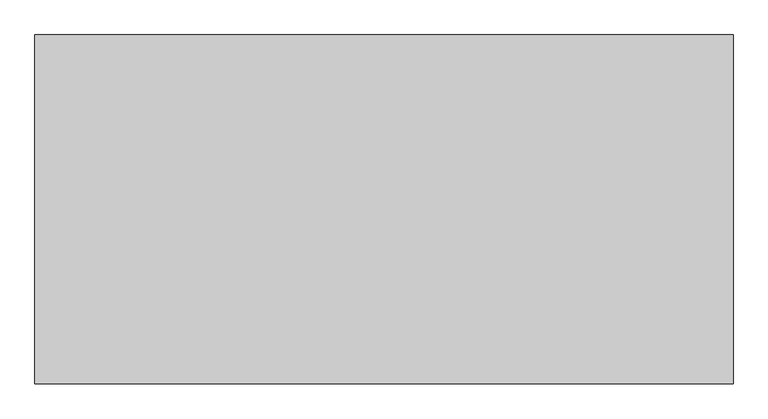
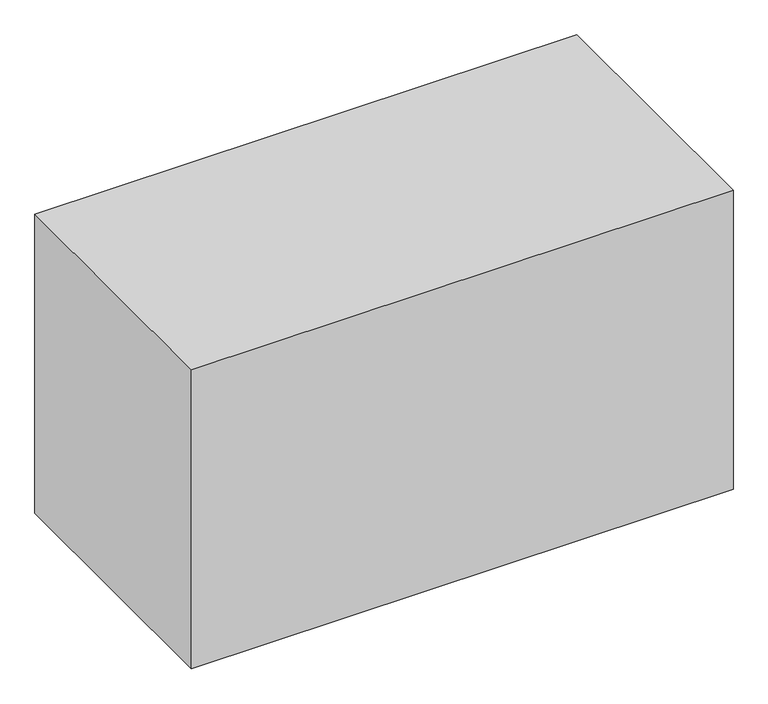
"""IFC4 building model written with IfcOpenShell, lengths in millimetres: proxy geometry, Space Planning Box_hec : Space Planning Box_hec."""

import ifcopenshell
import ifcopenshell.guid

model = None  # the IFC model being written
_history = None  # IfcOwnerHistory: only IFC2X3 demands one
_inside = {}  # id of a spatial element -> (the spatial element, [elements in it])
_under = {}  # id of a project, library or spatial element -> (it, [spatial elements below it])
_declared = {}  # id of a project -> (the project, [libraries it declares])
_typed = {}  # id of a type object -> (the type object, [elements of that type])
_made_of = {}  # id of a material, layer set ... -> (it, [elements and type objects made of it])


def new_model(schema):
    """Start an empty IFC model of exactly this schema.

    Asked for "IFC4X3", IfcOpenShell would pick the latest addendum, in which some entities
    have other attributes; the version numbers below select the first issue.
    IFC2X3 requires an IfcOwnerHistory on every rooted entity: one is made here for all.
    """
    global model, _history
    if schema == "IFC4X3":
        model = ifcopenshell.file(schema_version=(4, 3, 0, 0))
    else:
        model = ifcopenshell.file(schema=schema)
    _inside.clear()
    _under.clear()
    _declared.clear()
    _typed.clear()
    _made_of.clear()
    _history = None
    if model.schema == "IFC2X3":
        org = make("IfcOrganization", Name="unknown")
        user = make(
            "IfcPersonAndOrganization",
            ThePerson=make("IfcPerson", FamilyName="unknown"),
            TheOrganization=org,
        )
        app = make(
            "IfcApplication",
            ApplicationDeveloper=org,
            Version="unknown",
            ApplicationFullName="unknown",
            ApplicationIdentifier="unknown",
        )
        _history = make(
            "IfcOwnerHistory",
            OwningUser=user,
            OwningApplication=app,
            ChangeAction="ADDED",
            CreationDate=0,
        )
    return model


def make(cls, **values):
    """One entity of the class cls with the attributes given. An attribute that is None is left unset."""
    return model.create_entity(
        cls, **{name: value for name, value in values.items() if value is not None}
    )


def rooted(cls, **values):
    """An entity with a GlobalId (a new one), such as an element, a storey or a relation."""
    return make(cls, GlobalId=ifcopenshell.guid.new(), OwnerHistory=_history, **values)


def si_unit(unit_type, name, prefix=None):
    """IfcSIUnit, for example si_unit("LENGTHUNIT", "METRE", prefix="MILLI")."""
    return make("IfcSIUnit", UnitType=unit_type, Prefix=prefix, Name=name)


def assignment(units):
    """IfcUnitAssignment: the units of a project."""
    return None if units is None else make("IfcUnitAssignment", Units=units)


def point(xyz):
    """IfcCartesianPoint."""
    return None if xyz is None else make("IfcCartesianPoint", Coordinates=xyz)


def direction(xyz):
    """IfcDirection."""
    return None if xyz is None else make("IfcDirection", DirectionRatios=xyz)


def frame(location, z_axis=None, x_axis=None):
    """IfcAxis2Placement3D, a coordinate frame: its origin and axes. An axis left out is left unset."""
    return make(
        "IfcAxis2Placement3D",
        Location=point(location),
        Axis=direction(z_axis),
        RefDirection=direction(x_axis),
    )


def origin():
    """The frame at (0, 0, 0) with its axes left unset."""
    return frame((0.0, 0.0, 0.0))


def origin_with_axes():
    """The frame at (0, 0, 0) with the z axis (0, 0, 1) and the x axis (1, 0, 0) written out."""
    return frame((0.0, 0.0, 0.0), z_axis=(0.0, 0.0, 1.0), x_axis=(1.0, 0.0, 0.0))


def place(relative_to, where):
    """IfcLocalPlacement: puts the frame where relative to a parent placement (None: the world)."""
    return make(
        "IfcLocalPlacement", PlacementRelTo=relative_to, RelativePlacement=where
    )


def context(
    kind, dimensions, precision=None, world=None, true_north=None, identifier=None
):
    """IfcGeometricRepresentationContext, for example the 3D "Model" context."""
    return make(
        "IfcGeometricRepresentationContext",
        ContextIdentifier=identifier,
        ContextType=kind,
        CoordinateSpaceDimension=dimensions,
        Precision=precision,
        WorldCoordinateSystem=world,
        TrueNorth=true_north,
    )


def project(units=None, contexts=None):
    """IfcProject with its units and contexts."""
    return rooted(
        "IfcProject",
        Name="project",
        RepresentationContexts=contexts,
        UnitsInContext=assignment(units),
    )


def spatial(cls, under=None, at=None, **own):
    """A site, building, storey or space (cls), placed at a placement, below another one or the project."""
    s = rooted(cls, ObjectPlacement=at, **own)
    if under is not None:
        _under.setdefault(under.id(), (under, []))[1].append(s)
    return s


def polyline(points):
    """IfcPolyline through the points."""
    return make("IfcPolyline", Points=[point(p) for p in points])


def outline(outer, holes=None, kind="AREA"):
    """IfcArbitraryClosedProfileDef: a profile drawn as a closed curve; with holes, ...WithVoids."""
    if holes is None:
        return make("IfcArbitraryClosedProfileDef", ProfileType=kind, OuterCurve=outer)
    return make(
        "IfcArbitraryProfileDefWithVoids",
        ProfileType=kind,
        OuterCurve=outer,
        InnerCurves=holes,
    )


def extrude(swept, where, along, depth):
    """IfcExtrudedAreaSolid: the profile swept, set in the frame where, extruded along a direction by depth."""
    return make(
        "IfcExtrudedAreaSolid",
        SweptArea=swept,
        Position=where,
        ExtrudedDirection=direction(along),
        Depth=depth,
    )


def shape(context_of_items, identifier, shape_type, items):
    """IfcShapeRepresentation: the items that make up one representation, for example the "Body"."""
    return make(
        "IfcShapeRepresentation",
        ContextOfItems=context_of_items,
        RepresentationIdentifier=identifier,
        RepresentationType=shape_type,
        Items=items,
    )


def source(mapping_origin, context_of_items, identifier, shape_type, items):
    """IfcRepresentationMap: a shape defined once, which mapped items show again and again."""
    return make(
        "IfcRepresentationMap",
        MappingOrigin=mapping_origin,
        MappedRepresentation=shape(context_of_items, identifier, shape_type, items),
    )


def transform(
    local_origin,
    x_axis=None,
    y_axis=None,
    z_axis=None,
    scale=None,
    scale2=None,
    scale3=None,
    uniform=True,
):
    """IfcCartesianTransformationOperator3D, or its non-uniform kind. x_axis, y_axis, z_axis: its Axis1, 2, 3."""
    if uniform:
        return make(
            "IfcCartesianTransformationOperator3D",
            Axis1=direction(x_axis),
            Axis2=direction(y_axis),
            LocalOrigin=point(local_origin),
            Scale=scale,
            Axis3=direction(z_axis),
        )
    return make(
        "IfcCartesianTransformationOperator3DnonUniform",
        Axis1=direction(x_axis),
        Axis2=direction(y_axis),
        LocalOrigin=point(local_origin),
        Scale=scale,
        Axis3=direction(z_axis),
        Scale2=scale2,
        Scale3=scale3,
    )


def mapped(mapping_source, mapping_target):
    """IfcMappedItem: shows the shape of a source again, moved by a transform."""
    return make(
        "IfcMappedItem", MappingSource=mapping_source, MappingTarget=mapping_target
    )


def made_of(thing, what):
    """Note that an element or type object is made of a material, layer set ...; save() writes the relation."""
    if what is not None:
        _made_of.setdefault(what.id(), (what, []))[1].append(thing)
    return thing


def element(
    cls,
    number,
    at=None,
    inside=None,
    cuts=None,
    type_object=None,
    material=None,
    context=None,
    identifier="Body",
    shape_type=None,
    held_by="IfcProductDefinitionShape",
    body=None,
    shapes=None,
    **own,
):
    """One element of the class cls, such as IfcWall. Its Tag is "e" and its number.

    at: its placement. inside: the storey or other place that contains it. cuts: it is an
    opening in that element (IfcRelVoidsElement). A single representation is given by context,
    identifier, shape_type and body (its items); several are given by shapes. held_by: the class
    of the entity that holds the representations. save() writes the other relations.
    """
    e = rooted(cls, Tag="e%d" % number, ObjectPlacement=at, **own)
    if body is not None:
        shapes = [shape(context, identifier, shape_type, body)]
    if shapes is not None:
        e.Representation = make(held_by, Representations=shapes)
    if inside is not None:
        _inside.setdefault(inside.id(), (inside, []))[1].append(e)
    if cuts is not None:
        rooted(
            "IfcRelVoidsElement", RelatingBuildingElement=cuts, RelatedOpeningElement=e
        )
    if type_object is not None:
        _typed.setdefault(type_object.id(), (type_object, []))[1].append(e)
    return made_of(e, material)


def aggregate(whole, parts):
    """IfcRelAggregates: a whole, such as a stair, and the parts it consists of."""
    return rooted("IfcRelAggregates", RelatingObject=whole, RelatedObjects=parts)


def save(model, path):
    """Write the relations noted so far, then the file.

    IfcRelAggregates (storeys below a building ...), IfcRelContainedInSpatialStructure (elements
    in a storey), IfcRelDefinesByType, IfcRelAssociatesMaterial and IfcRelDeclares: one each for
    every whole, place, type object, material and project.
    """
    for whole, parts in _under.values():
        aggregate(whole, parts)
    for where, things in _inside.values():
        rooted(
            "IfcRelContainedInSpatialStructure",
            RelatedElements=things,
            RelatingStructure=where,
        )
    for kind, things in _typed.values():
        rooted("IfcRelDefinesByType", RelatedObjects=things, RelatingType=kind)
    for what, things in _made_of.values():
        rooted("IfcRelAssociatesMaterial", RelatedObjects=things, RelatingMaterial=what)
    for by, libraries in _declared.values():
        rooted("IfcRelDeclares", RelatingContext=by, RelatedDefinitions=libraries)
    model.write(path)


def generic_models_a5818909(model_context):
    return source(origin(), model_context, "Body", "SweptSolid", [
        extrude(outline(polyline([(3000.0, 1500.0), (3000.0, -1500.0), (-3000.0, -1500.0), (-3000.0, 1500.0), (3000.0, 1500.0)])), origin_with_axes(), (0.0, 0.0, 1.0), 3500.0),
    ])


if __name__ == "__main__":
    model = new_model("IFC4")
    model_context = context("Model", 3, world=origin())
    ifc_project = project(units=[si_unit("LENGTHUNIT", "METRE", prefix="MILLI")], contexts=[model_context])
    site = spatial("IfcSite", under=ifc_project)
    building = spatial("IfcBuilding", under=site)
    placement = place(None, origin())
    generic_models_shape = generic_models_a5818909(model_context)
    element("IfcBuildingElementProxy", 1, Name="Space Planning Box_hec : Space Planning Box_hec", ObjectType="Space Planning Box_hec : Space Planning Box_hec", at=placement, inside=building, context=model_context, shape_type="MappedRepresentation", body=[
        mapped(generic_models_shape, transform((0.0, 0.0, 0.0), x_axis=(1.0, 0.0, 0.0), y_axis=(0.0, 1.0, 0.0), z_axis=(0.0, 0.0, 1.0))),
    ])
    save(model, "model.ifc")

# Revit data of these elements
# Type "Space Planning Box_hec : Space Planning Box_hec"
#   Type Comments = "..."
#   Room Name [instance default] = "?"
#   Interior Finish [instance default] = ""
#   Exterior Finish [instance default] = ""
#   Department [instance default] = ""
#   Assembly Code = "..."
#   ceiling height [instance default] = 0
#   Width [instance default] = 1524 mm
#   Program Area [instance default] = 0.00 m²
#   Length [instance default] = 1524 mm
#   Height [instance default] = 1524 mm
#   Area [instance default] = 2.32258 m²
#   Fill Color [instance default] = Cyan
#   Default Elevation = 0
# Element 1 (IfcBuildingElementProxy, "Space Planning Box_hec : Space Planning Box_hec")
#   Room Name = "Locker(M)"
#   Exterior Finish = "RF1..N/A,,EW1..N/A..N/A"
#   Department = "AR"
#   Width = 6000 mm
#   Program Area = 18.00 m²
#   Length = 3000 mm
#   Height = 3500 mm
#   Area = 18.00 m²
#   Materials on its faces: "Cyan"
# Materials
#   "Cyan": class "Generic", colour RGB 0 255 255, transparency 0.2, Cost = 0
